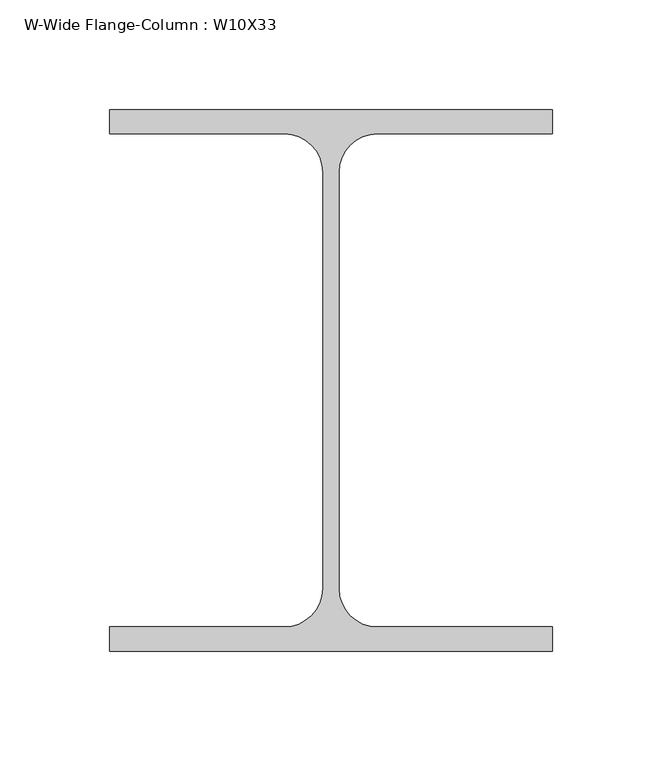
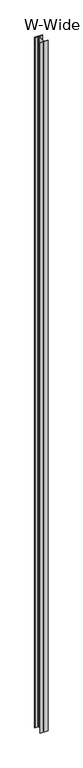
"""IFC4 building model written with IfcOpenShell, lengths in millimetres: column geometry, W-Wide Flange-Column : W10X33."""

from ifc_helpers import new_model, si_unit, point, frame, frame_2d, origin, place, context, project, spatial, polyline, circle_curve, trimmed, segment, composite_curve, outline, extrude, source, transform, mapped, element, save


def w_wide_flange_column_w10x33_2b06d58e(model_context):
    return source(origin(), model_context, "Body", "SweptSolid", [
        extrude(outline(composite_curve([segment(polyline([(101.092, 123.571), (101.092, 112.522), (21.209, 112.522)]), True, "CONTINUOUS"), segment(trimmed(circle_curve(frame_2d((21.209, 94.996)), 17.526), [point((21.209, 112.522))], [point((3.683, 94.996))], True, "CARTESIAN"), True, "CONTINUOUS"), segment(polyline([(3.683, 94.996), (3.683, -94.996)]), True, "CONTINUOUS"), segment(trimmed(circle_curve(frame_2d((21.209, -94.996)), 17.526), [point((3.683, -94.996))], [point((21.209, -112.522))], True, "CARTESIAN"), True, "CONTINUOUS"), segment(polyline([(21.209, -112.522), (101.092, -112.522), (101.092, -123.571), (-101.092, -123.571), (-101.092, -112.522), (-21.209, -112.522)]), True, "CONTINUOUS"), segment(trimmed(circle_curve(frame_2d((-21.209, -94.996)), 17.526), [point((-21.209, -112.522))], [point((-3.683, -94.996))], True, "CARTESIAN"), True, "CONTINUOUS"), segment(polyline([(-3.683, -94.996), (-3.683, 94.996)]), True, "CONTINUOUS"), segment(trimmed(circle_curve(frame_2d((-21.209, 94.996)), 17.526), [point((-3.683, 94.996))], [point((-21.209, 112.522))], True, "CARTESIAN"), True, "CONTINUOUS"), segment(polyline([(-21.209, 112.522), (-101.092, 112.522), (-101.092, 123.571), (101.092, 123.571)]), True, "CONTINUOUS")], self_intersect=False)), frame((0.0, 0.0, 8655.05), z_axis=(0.0, 0.0, 1.0), x_axis=(1.0, 0.0, 0.0)), (0.0, 0.0, 1.0), 18929.35),
    ])


if __name__ == "__main__":
    model = new_model("IFC4")
    model_context = context("Model", 3, world=origin())
    ifc_project = project(units=[si_unit("LENGTHUNIT", "METRE", prefix="MILLI")], contexts=[model_context])
    site = spatial("IfcSite", under=ifc_project)
    building = spatial("IfcBuilding", under=site)
    placement = place(None, origin())
    w_wide_flange_column_w10x33_shape = w_wide_flange_column_w10x33_2b06d58e(model_context)
    element("IfcColumn", 1, ObjectType="W-Wide Flange-Column : W10X33", at=placement, inside=building, context=model_context, shape_type="MappedRepresentation", body=[
        mapped(w_wide_flange_column_w10x33_shape, transform((0.0, 0.0, 0.0), x_axis=(1.0, 0.0, 0.0), y_axis=(0.0, 1.0, 0.0), z_axis=(0.0, 0.0, 1.0))),
    ])
    save(model, "model.ifc")

# Revit data of these elements
# Type "W-Wide Flange-Column : W10X33"
#   Assembly Code = "B10"
#   W = 33
#   bf = 0' - 7.96"
#   d = 0' - 9.73"
#   k = 0' - 1 1/8"
#   kr = 0' - 0.69"
#   tf = 0' - 0.435"
#   tw = 0' - 0.29"
#   A = 0.0674306 SF
#   Structural Material [instance default] = Steel ASTM A992
# Element 1 (IfcColumn, "W-Wide Flange-Column : W10X33")
#   Materials on its faces: "Steel ASTM A992"
# Materials
#   "Steel ASTM A992": class "Metal", colour RGB 199 199 199, transparency 0, Description = "Structural steel 50ksi", Cost = 0
